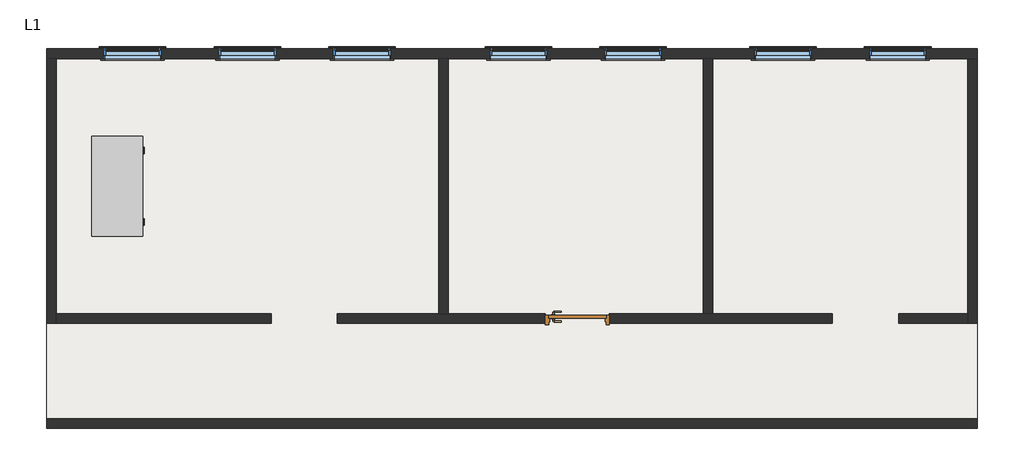
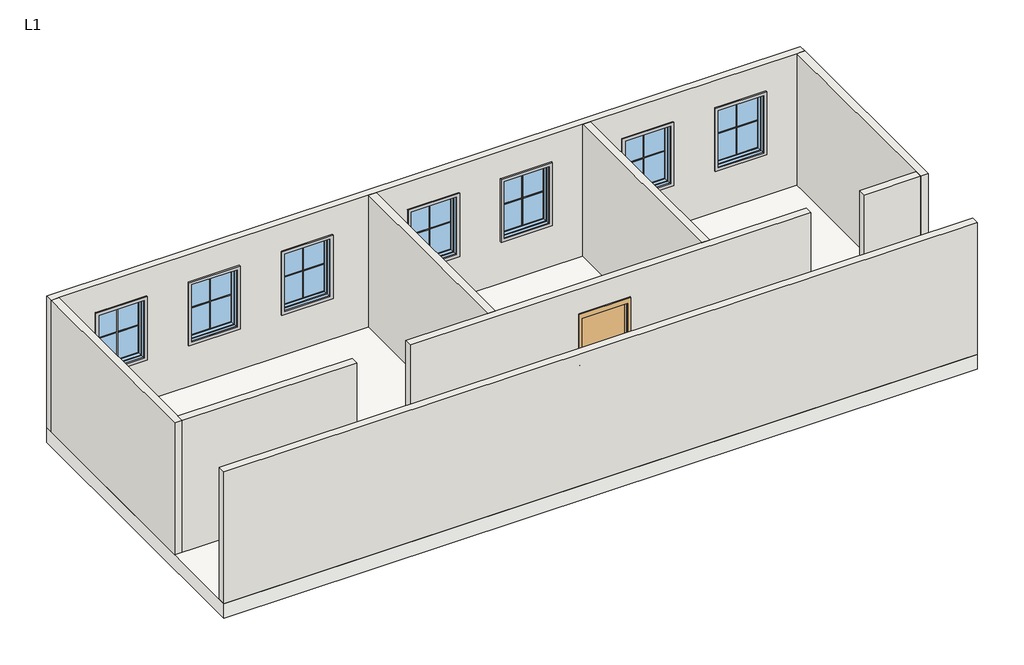
# One storey: 21 proxies, 9 walls, 7 windows, 1 door, 1 furniture element, 1 slab.
"""IFC4 building model written with IfcOpenShell, lengths in millimetres."""

import ifcopenshell
import ifcopenshell.guid

model = None  # the IFC model being written
_history = None  # IfcOwnerHistory: only IFC2X3 demands one
_inside = {}  # id of a spatial element -> (the spatial element, [elements in it])
_under = {}  # id of a project, library or spatial element -> (it, [spatial elements below it])
_declared = {}  # id of a project -> (the project, [libraries it declares])
_typed = {}  # id of a type object -> (the type object, [elements of that type])
_made_of = {}  # id of a material, layer set ... -> (it, [elements and type objects made of it])


def new_model(schema):
    """Start an empty IFC model of exactly this schema.

    Asked for "IFC4X3", IfcOpenShell would pick the latest addendum, in which some entities
    have other attributes; the version numbers below select the first issue.
    IFC2X3 requires an IfcOwnerHistory on every rooted entity: one is made here for all.
    """
    global model, _history
    if schema == "IFC4X3":
        model = ifcopenshell.file(schema_version=(4, 3, 0, 0))
    else:
        model = ifcopenshell.file(schema=schema)
    _inside.clear()
    _under.clear()
    _declared.clear()
    _typed.clear()
    _made_of.clear()
    _history = None
    if model.schema == "IFC2X3":
        org = make("IfcOrganization", Name="unknown")
        user = make(
            "IfcPersonAndOrganization",
            ThePerson=make("IfcPerson", FamilyName="unknown"),
            TheOrganization=org,
        )
        app = make(
            "IfcApplication",
            ApplicationDeveloper=org,
            Version="unknown",
            ApplicationFullName="unknown",
            ApplicationIdentifier="unknown",
        )
        _history = make(
            "IfcOwnerHistory",
            OwningUser=user,
            OwningApplication=app,
            ChangeAction="ADDED",
            CreationDate=0,
        )
    return model


def make(cls, **values):
    """One entity of the class cls with the attributes given. An attribute that is None is left unset."""
    return model.create_entity(
        cls, **{name: value for name, value in values.items() if value is not None}
    )


def rooted(cls, **values):
    """An entity with a GlobalId (a new one), such as an element, a storey or a relation."""
    return make(cls, GlobalId=ifcopenshell.guid.new(), OwnerHistory=_history, **values)


def si_unit(unit_type, name, prefix=None):
    """IfcSIUnit, for example si_unit("LENGTHUNIT", "METRE", prefix="MILLI")."""
    return make("IfcSIUnit", UnitType=unit_type, Prefix=prefix, Name=name)


def assignment(units):
    """IfcUnitAssignment: the units of a project."""
    return None if units is None else make("IfcUnitAssignment", Units=units)


def point(xyz):
    """IfcCartesianPoint."""
    return None if xyz is None else make("IfcCartesianPoint", Coordinates=xyz)


def direction(xyz):
    """IfcDirection."""
    return None if xyz is None else make("IfcDirection", DirectionRatios=xyz)


def frame(location, z_axis=None, x_axis=None):
    """IfcAxis2Placement3D, a coordinate frame: its origin and axes. An axis left out is left unset."""
    return make(
        "IfcAxis2Placement3D",
        Location=point(location),
        Axis=direction(z_axis),
        RefDirection=direction(x_axis),
    )


def frame_2d(location, x_axis=None):
    """IfcAxis2Placement2D, a coordinate frame in the plane: its origin and x axis."""
    return make(
        "IfcAxis2Placement2D", Location=point(location), RefDirection=direction(x_axis)
    )


def origin():
    """The frame at (0, 0, 0) with its axes left unset."""
    return frame((0.0, 0.0, 0.0))


def origin_with_axes():
    """The frame at (0, 0, 0) with the z axis (0, 0, 1) and the x axis (1, 0, 0) written out."""
    return frame((0.0, 0.0, 0.0), z_axis=(0.0, 0.0, 1.0), x_axis=(1.0, 0.0, 0.0))


def place(relative_to, where):
    """IfcLocalPlacement: puts the frame where relative to a parent placement (None: the world)."""
    return make(
        "IfcLocalPlacement", PlacementRelTo=relative_to, RelativePlacement=where
    )


def context(
    kind, dimensions, precision=None, world=None, true_north=None, identifier=None
):
    """IfcGeometricRepresentationContext, for example the 3D "Model" context."""
    return make(
        "IfcGeometricRepresentationContext",
        ContextIdentifier=identifier,
        ContextType=kind,
        CoordinateSpaceDimension=dimensions,
        Precision=precision,
        WorldCoordinateSystem=world,
        TrueNorth=true_north,
    )


def project(units=None, contexts=None):
    """IfcProject with its units and contexts."""
    return rooted(
        "IfcProject",
        Name="project",
        RepresentationContexts=contexts,
        UnitsInContext=assignment(units),
    )


def spatial(cls, under=None, at=None, **own):
    """A site, building, storey or space (cls), placed at a placement, below another one or the project."""
    s = rooted(cls, ObjectPlacement=at, **own)
    if under is not None:
        _under.setdefault(under.id(), (under, []))[1].append(s)
    return s


def polyline(points):
    """IfcPolyline through the points."""
    return make("IfcPolyline", Points=[point(p) for p in points])


def circle_curve(where, radius):
    """IfcCircle in the frame where."""
    return make("IfcCircle", Position=where, Radius=radius)


def ellipse_curve(where, semi_axis1, semi_axis2):
    """IfcEllipse in the frame where."""
    return make(
        "IfcEllipse", Position=where, SemiAxis1=semi_axis1, SemiAxis2=semi_axis2
    )


def trimmed(basis, trim1, trim2, sense, master):
    """IfcTrimmedCurve: the piece of a basis curve between two trims."""
    return make(
        "IfcTrimmedCurve",
        BasisCurve=basis,
        Trim1=trim1,
        Trim2=trim2,
        SenseAgreement=sense,
        MasterRepresentation=master,
    )


def segment(curve, same_sense, transition):
    """IfcCompositeCurveSegment."""
    return make(
        "IfcCompositeCurveSegment",
        Transition=transition,
        SameSense=same_sense,
        ParentCurve=curve,
    )


def composite_curve(segments, self_intersect=None):
    """IfcCompositeCurve: segments joined end to end."""
    return make("IfcCompositeCurve", Segments=segments, SelfIntersect=self_intersect)


def outline(outer, holes=None, kind="AREA"):
    """IfcArbitraryClosedProfileDef: a profile drawn as a closed curve; with holes, ...WithVoids."""
    if holes is None:
        return make("IfcArbitraryClosedProfileDef", ProfileType=kind, OuterCurve=outer)
    return make(
        "IfcArbitraryProfileDefWithVoids",
        ProfileType=kind,
        OuterCurve=outer,
        InnerCurves=holes,
    )


def extrude(swept, where, along, depth):
    """IfcExtrudedAreaSolid: the profile swept, set in the frame where, extruded along a direction by depth."""
    return make(
        "IfcExtrudedAreaSolid",
        SweptArea=swept,
        Position=where,
        ExtrudedDirection=direction(along),
        Depth=depth,
    )


def faces_of(points, faces, orient=None, outer=None):
    """IfcFace entities. A face is a list of loops; a loop is a list of indices into points, from 0.

    orient and outer hold one flag for each loop. By default every Orientation is true, the
    first loop of a face is its IfcFaceOuterBound and the others are IfcFaceBound.
    """
    made = []
    for i, loops in enumerate(faces):
        bounds = []
        for j, loop in enumerate(loops):
            is_outer = j == 0 if outer is None else outer[i][j]
            bounds.append(
                make(
                    "IfcFaceOuterBound" if is_outer else "IfcFaceBound",
                    Bound=make("IfcPolyLoop", Polygon=[points[k] for k in loop]),
                    Orientation=True if orient is None else orient[i][j],
                )
            )
        made.append(make("IfcFace", Bounds=bounds))
    return made


def faceted_brep(points, faces, orient=None, outer=None, voids=None):
    """IfcFacetedBrep: a solid bounded by flat faces; with voids (closed shells), ...WithVoids."""
    shared = [point(p) for p in points]
    hull = make("IfcClosedShell", CfsFaces=faces_of(shared, faces, orient, outer))
    if voids is None:
        return make("IfcFacetedBrep", Outer=hull)
    return make(
        "IfcFacetedBrepWithVoids",
        Outer=hull,
        Voids=[
            make(cls, CfsFaces=faces_of(shared, fs, o, b)) for cls, fs, o, b in voids
        ],
    )


def shape(context_of_items, identifier, shape_type, items):
    """IfcShapeRepresentation: the items that make up one representation, for example the "Body"."""
    return make(
        "IfcShapeRepresentation",
        ContextOfItems=context_of_items,
        RepresentationIdentifier=identifier,
        RepresentationType=shape_type,
        Items=items,
    )


def source(mapping_origin, context_of_items, identifier, shape_type, items):
    """IfcRepresentationMap: a shape defined once, which mapped items show again and again."""
    return make(
        "IfcRepresentationMap",
        MappingOrigin=mapping_origin,
        MappedRepresentation=shape(context_of_items, identifier, shape_type, items),
    )


def transform(
    local_origin,
    x_axis=None,
    y_axis=None,
    z_axis=None,
    scale=None,
    scale2=None,
    scale3=None,
    uniform=True,
):
    """IfcCartesianTransformationOperator3D, or its non-uniform kind. x_axis, y_axis, z_axis: its Axis1, 2, 3."""
    if uniform:
        return make(
            "IfcCartesianTransformationOperator3D",
            Axis1=direction(x_axis),
            Axis2=direction(y_axis),
            LocalOrigin=point(local_origin),
            Scale=scale,
            Axis3=direction(z_axis),
        )
    return make(
        "IfcCartesianTransformationOperator3DnonUniform",
        Axis1=direction(x_axis),
        Axis2=direction(y_axis),
        LocalOrigin=point(local_origin),
        Scale=scale,
        Axis3=direction(z_axis),
        Scale2=scale2,
        Scale3=scale3,
    )


def mapped(mapping_source, mapping_target):
    """IfcMappedItem: shows the shape of a source again, moved by a transform."""
    return make(
        "IfcMappedItem", MappingSource=mapping_source, MappingTarget=mapping_target
    )


def made_of(thing, what):
    """Note that an element or type object is made of a material, layer set ...; save() writes the relation."""
    if what is not None:
        _made_of.setdefault(what.id(), (what, []))[1].append(thing)
    return thing


def element(
    cls,
    number,
    at=None,
    inside=None,
    cuts=None,
    type_object=None,
    material=None,
    context=None,
    identifier="Body",
    shape_type=None,
    held_by="IfcProductDefinitionShape",
    body=None,
    shapes=None,
    **own,
):
    """One element of the class cls, such as IfcWall. Its Tag is "e" and its number.

    at: its placement. inside: the storey or other place that contains it. cuts: it is an
    opening in that element (IfcRelVoidsElement). A single representation is given by context,
    identifier, shape_type and body (its items); several are given by shapes. held_by: the class
    of the entity that holds the representations. save() writes the other relations.
    """
    e = rooted(cls, Tag="e%d" % number, ObjectPlacement=at, **own)
    if body is not None:
        shapes = [shape(context, identifier, shape_type, body)]
    if shapes is not None:
        e.Representation = make(held_by, Representations=shapes)
    if inside is not None:
        _inside.setdefault(inside.id(), (inside, []))[1].append(e)
    if cuts is not None:
        rooted(
            "IfcRelVoidsElement", RelatingBuildingElement=cuts, RelatedOpeningElement=e
        )
    if type_object is not None:
        _typed.setdefault(type_object.id(), (type_object, []))[1].append(e)
    return made_of(e, material)


def aggregate(whole, parts):
    """IfcRelAggregates: a whole, such as a stair, and the parts it consists of."""
    return rooted("IfcRelAggregates", RelatingObject=whole, RelatedObjects=parts)


def save(model, path):
    """Write the relations noted so far, then the file.

    IfcRelAggregates (storeys below a building ...), IfcRelContainedInSpatialStructure (elements
    in a storey), IfcRelDefinesByType, IfcRelAssociatesMaterial and IfcRelDeclares: one each for
    every whole, place, type object, material and project.
    """
    for whole, parts in _under.values():
        aggregate(whole, parts)
    for where, things in _inside.values():
        rooted(
            "IfcRelContainedInSpatialStructure",
            RelatedElements=things,
            RelatingStructure=where,
        )
    for kind, things in _typed.values():
        rooted("IfcRelDefinesByType", RelatedObjects=things, RelatingType=kind)
    for what, things in _made_of.values():
        rooted("IfcRelAssociatesMaterial", RelatedObjects=things, RelatingMaterial=what)
    for by, libraries in _declared.values():
        rooted("IfcRelDeclares", RelatingContext=by, RelatedDefinitions=libraries)
    model.write(path)


def plane_surface(at):
    """IfcPlane: the flat surface through the origin of the frame at, square to its z axis."""
    return make("IfcPlane", Position=at)


def cylinder_surface(at, radius):
    """IfcCylindricalSurface: all points at the distance radius from the z axis of the frame at."""
    return make("IfcCylindricalSurface", Position=at, Radius=radius)


def revolved_surface(curve, axis_point, axis_direction):
    """IfcSurfaceOfRevolution: the curve turned about the line through axis_point along axis_direction."""
    return make(
        "IfcSurfaceOfRevolution",
        SweptCurve=make("IfcArbitraryOpenProfileDef", ProfileType="CURVE", Curve=curve),
        AxisPosition=make("IfcAxis1Placement", Location=point(axis_point), Axis=direction(axis_direction)),
    )


def advanced_brep(points, edges, surfaces, faces):
    """IfcAdvancedBrep: a solid bounded by faces that lie on surfaces and meet in shared edges.

    An edge is (start, end): straight between two places in points (the first is 0);
    or (start, end, curve); or (start, end, curve, False) where it runs against its curve.
    A face is (place in surfaces, loops), or (place, loops, False) where it looks against
    its surface's normal. A loop lists edges by number (the first is 1), with a minus sign
    where the edge is run from its end to its start. The first loop is the outer one.
    """
    corners = [point(p) for p in points]
    vertices = [make("IfcVertexPoint", VertexGeometry=c) for c in corners]
    made = []
    for start, end, *more in edges:
        made.append(
            make(
                "IfcEdgeCurve",
                EdgeStart=vertices[start],
                EdgeEnd=vertices[end],
                EdgeGeometry=more[0] if more else make("IfcPolyline", Points=[corners[start], corners[end]]),
                SameSense=more[1] if len(more) > 1 else True,
            )
        )
    hull = []
    for where, loops, *sense in faces:
        bounds = []
        for j, loop in enumerate(loops):
            ring = [make("IfcOrientedEdge", EdgeElement=made[abs(k) - 1], Orientation=k > 0) for k in loop]
            bounds.append(
                make(
                    "IfcFaceOuterBound" if j == 0 else "IfcFaceBound",
                    Bound=make("IfcEdgeLoop", EdgeList=ring),
                    Orientation=True,
                )
            )
        hull.append(make("IfcAdvancedFace", Bounds=bounds, FaceSurface=surfaces[where], SameSense=sense[0] if sense else True))
    return make("IfcAdvancedBrep", Outer=make("IfcClosedShell", CfsFaces=hull))


def m_muntin_pattern_2x2_m_muntin_pattern_2x2_ad852c99(model_context):
    return source(origin(), model_context, "Body", "SweptSolid", [
        extrude(outline(polyline([(568.25, -6.35), (568.25, -411.9), (555.55, -411.9), (555.55, -6.35), (0.0, -6.35), (0.0, 6.35), (555.55, 6.35), (555.55, 411.9), (568.25, 411.9), (568.25, 6.35), (1123.8, 6.35), (1123.8, -6.35), (568.25, -6.35)])), frame((0.0, -22.225, 0.0), z_axis=(0.0, 1.0, 0.0), x_axis=(0.0, 0.0, 1.0)), (0.0, 0.0, 1.0), 12.7),
        extrude(outline(polyline([(568.25, -6.35), (568.25, -411.9), (555.55, -411.9), (555.55, -6.35), (0.0, -6.35), (0.0, 6.35), (555.55, 6.35), (555.55, 411.9), (568.25, 411.9), (568.25, 6.35), (1123.8, 6.35), (1123.8, -6.35), (568.25, -6.35)])), frame((0.0, 9.525, 0.0), z_axis=(0.0, 1.0, 0.0), x_axis=(0.0, 0.0, 1.0)), (0.0, 0.0, 1.0), 12.7),
    ])


def m_trim_window_exterior_flat_with_sill_71544b40(model_context):
    return source(origin(), model_context, "Body", "SweptSolid", [
        extrude(outline(polyline([(510.0, -1220.4323709), (510.0, -1280.4323709), (-510.0, -1280.4323709), (-510.0, -1220.4323709), (510.0, -1220.4323709)])), origin_with_axes(), (0.0, 0.0, 1.0), 19.05),
        extrude(outline(polyline([(-1230.0, 38.1), (-1202.4580645, 38.1), (-1200.0, 19.05), (-1200.0, 0.0), (-1220.4323709, 0.0), (-1220.4323709, 19.05), (-1230.0, 19.05), (-1230.0, 38.1)])), frame((-522.7, 0.0, 0.0), z_axis=(1.0, 0.0, 0.0), x_axis=(0.0, 1.0, 0.0)), (0.0, 0.0, 1.0), 1045.4),
        extrude(outline(polyline([(-510.0, 60.0), (510.0, 60.0), (510.0, -1200.0), (450.0, -1200.0), (450.0, 0.0), (-450.0, 0.0), (-450.0, -1200.0), (-510.0, -1200.0), (-510.0, 60.0)])), origin_with_axes(), (0.0, 0.0, 1.0), 19.05),
    ])


def m_trim_window_interior_flat_picture_frame_24fe8ef8(model_context):
    return source(origin(), model_context, "Body", "SweptSolid", [
        extrude(outline(polyline([(497.3, 47.3), (497.3, -1247.3), (-497.3, -1247.3), (-497.3, 47.3), (497.3, 47.3)]), holes=[polyline([(437.3, -12.7), (-437.3, -12.7), (-437.3, -1187.3), (437.3, -1187.3), (437.3, -12.7)])]), origin_with_axes(), (0.0, 0.0, 1.0), 30.0),
    ])


def m_door_passage_single_flush_900_x_2100mm_f70d95c9(model_context):
    return source(origin(), model_context, "Body", "SolidModel", [
        advanced_brep(
        [(-384.990625, 3.35, 1000.0), (-364.990625, 3.35, 1000.0), (-364.990625, -26.65, 1000.0), (-384.990625, -26.65, 1000.0), (-359.990625, -31.65, 1000.0), (-359.990625, -51.65, 1000.0), (-254.990625, -51.65, 1000.0), (-254.990625, -31.65, 1000.0)],
        [
            (0, 1, circle_curve(frame((-374.990625, 3.35, 1000.0), z_axis=(0.0, 1.0, 0.0), x_axis=(1.0, 0.0, 0.0)), 10.0)),
            (1, 0, circle_curve(frame((-374.990625, 3.35, 1000.0), z_axis=(0.0, 1.0, 0.0), x_axis=(1.0, 0.0, 0.0)), 10.0)),
            (1, 2),
            (2, 3, circle_curve(frame((-374.990625, -26.65, 1000.0), z_axis=(0.0, 1.0, 0.0), x_axis=(1.0, 0.0, 0.0)), 10.0)),
            (3, 0),
            (3, 2, circle_curve(frame((-374.990625, -26.65, 1000.0), z_axis=(0.0, 1.0, 0.0), x_axis=(1.0, 0.0, 0.0)), 10.0)),
            (4, 5, circle_curve(frame((-359.990625, -41.65, 1000.0), z_axis=(-1.0, 0.0, 0.0), x_axis=(0.0, 1.0, 0.0)), 10.0)),
            (5, 3, circle_curve(frame((-359.990625, -26.65, 1000.0), z_axis=(0.0, 0.0, -1.0), x_axis=(-1.0, 0.0, 0.0)), 25.0)),
            (2, 4, circle_curve(frame((-359.990625, -26.65, 1000.0), z_axis=(0.0, 0.0, 1.0), x_axis=(-1.0, 0.0, 0.0)), 5.0)),
            (5, 4, circle_curve(frame((-359.990625, -41.65, 1000.0), z_axis=(-1.0, 0.0, 0.0), x_axis=(0.0, 1.0, 0.0)), 10.0)),
            (6, 7, circle_curve(frame((-254.990625, -41.65, 1000.0), z_axis=(1.0, 0.0, 0.0), x_axis=(0.0, 1.0, 0.0)), 10.0)),
            (7, 6, circle_curve(frame((-254.990625, -41.65, 1000.0), z_axis=(1.0, 0.0, 0.0), x_axis=(0.0, 1.0, 0.0)), 10.0)),
            (4, 7),
            (6, 5),
        ],
        [
            plane_surface(frame((-374.990625, 3.35, 1000.0), z_axis=(0.0, 1.0, 0.0), x_axis=(0.0, 0.0, 1.0))),
            cylinder_surface(frame((-374.990625, 3.35, 1000.0), z_axis=(0.0, 1.0, 0.0), x_axis=(1.0, 0.0, 0.0)), 10.0),
            revolved_surface(trimmed(ellipse_curve(frame((-374.990625, -26.65, 1000.0), z_axis=(0.0, -1.0, 0.0), x_axis=(1.0, 0.0, 0.0)), 10.0, 10.0), [point((-384.990625, -26.65, 1000.0))], [point((-364.990625, -26.65, 1000.0))], True, "CARTESIAN"), (-359.990625, -26.65, 1000.0), (0.0, 0.0, -1.0)),
            revolved_surface(trimmed(ellipse_curve(frame((-374.990625, -26.65, 1000.0), z_axis=(0.0, -1.0, 0.0), x_axis=(1.0, 0.0, 0.0)), 10.0, 10.0), [point((-364.990625, -26.65, 1000.0))], [point((-384.990625, -26.65, 1000.0))], True, "CARTESIAN"), (-359.990625, -26.65, 1000.0), (0.0, 0.0, -1.0)),
            plane_surface(frame((-254.990625, -41.65, 1000.0), z_axis=(1.0, 0.0, 0.0), x_axis=(0.0, 0.0, 1.0))),
            cylinder_surface(frame((-359.990625, -41.65, 1000.0), z_axis=(-1.0, 0.0, 0.0), x_axis=(0.0, 1.0, 0.0)), 10.0),
        ],
        [
            (0, [[1, 2]]),
            (1, [[3, 4, 5, -2]]),
            (1, [[-5, 6, -3, -1]]),
            (2, [[7, 8, -4, 9]]),
            (3, [[10, -9, -6, -8]]),
            (4, [[11, 12]]),
            (5, [[13, -11, 14, -7]]),
            (5, [[-14, -12, -13, -10]]),
        ],
    ),
        extrude(outline(composite_curve([segment(trimmed(circle_curve(frame_2d((1000.0, -377.490625)), 30.0), [point((1000.0, -407.490625))], [point((1000.0, -347.490625))], False, "CARTESIAN"), True, "CONTINUOUS"), segment(trimmed(circle_curve(frame_2d((1000.0, -377.490625)), 30.0), [point((1000.0, -347.490625))], [point((1000.0, -407.490625))], False, "CARTESIAN"), True, "CONTINUOUS")], self_intersect=False)), frame((0.0, 3.35, 0.0), z_axis=(0.0, 1.0, 0.0), x_axis=(0.0, 0.0, 1.0)), (0.0, 0.0, 1.0), 8.0),
        advanced_brep(
        [(-384.990625, 64.35, 1000.0), (-364.990625, 64.35, 1000.0), (-384.990625, 94.35, 1000.0), (-364.990625, 94.35, 1000.0), (-359.990625, 99.35, 1000.0), (-359.990625, 119.35, 1000.0), (-254.990625, 119.35, 1000.0), (-254.990625, 99.35, 1000.0)],
        [
            (0, 1, circle_curve(frame((-374.990625, 64.35, 1000.0), z_axis=(0.0, -1.0, 0.0), x_axis=(1.0, 0.0, 0.0)), 10.0)),
            (1, 0, circle_curve(frame((-374.990625, 64.35, 1000.0), z_axis=(0.0, -1.0, 0.0), x_axis=(1.0, 0.0, 0.0)), 10.0)),
            (0, 2),
            (2, 3, circle_curve(frame((-374.990625, 94.35, 1000.0), z_axis=(0.0, -1.0, 0.0), x_axis=(1.0, 0.0, 0.0)), 10.0)),
            (3, 1),
            (3, 2, circle_curve(frame((-374.990625, 94.35, 1000.0), z_axis=(0.0, -1.0, 0.0), x_axis=(1.0, 0.0, 0.0)), 10.0)),
            (4, 3, circle_curve(frame((-359.990625, 94.35, 1000.0), z_axis=(0.0, 0.0, 1.0), x_axis=(-1.0, 0.0, 0.0)), 5.0)),
            (2, 5, circle_curve(frame((-359.990625, 94.35, 1000.0), z_axis=(0.0, 0.0, -1.0), x_axis=(-1.0, 0.0, 0.0)), 25.0)),
            (5, 4, circle_curve(frame((-359.990625, 109.35, 1000.0), z_axis=(-1.0, 0.0, 0.0), x_axis=(0.0, -1.0, 0.0)), 10.0)),
            (4, 5, circle_curve(frame((-359.990625, 109.35, 1000.0), z_axis=(-1.0, 0.0, 0.0), x_axis=(0.0, -1.0, 0.0)), 10.0)),
            (6, 7, circle_curve(frame((-254.990625, 109.35, 1000.0), z_axis=(1.0, 0.0, 0.0), x_axis=(0.0, -1.0, 0.0)), 10.0)),
            (7, 6, circle_curve(frame((-254.990625, 109.35, 1000.0), z_axis=(1.0, 0.0, 0.0), x_axis=(0.0, -1.0, 0.0)), 10.0)),
            (5, 6),
            (7, 4),
        ],
        [
            plane_surface(frame((-374.990625, 64.35, 1000.0), z_axis=(0.0, -1.0, 0.0), x_axis=(0.0, 0.0, 1.0))),
            cylinder_surface(frame((-374.990625, 64.35, 1000.0), z_axis=(0.0, -1.0, 0.0), x_axis=(1.0, 0.0, 0.0)), 10.0),
            revolved_surface(trimmed(ellipse_curve(frame((-374.990625, 94.35, 1000.0), z_axis=(0.0, -1.0, 0.0), x_axis=(1.0, 0.0, 0.0)), 10.0, 10.0), [point((-384.990625, 94.35, 1000.0))], [point((-364.990625, 94.35, 1000.0))], True, "CARTESIAN"), (-359.990625, 94.35, 1000.0), (0.0, 0.0, -1.0)),
            revolved_surface(trimmed(ellipse_curve(frame((-374.990625, 94.35, 1000.0), z_axis=(0.0, -1.0, 0.0), x_axis=(1.0, 0.0, 0.0)), 10.0, 10.0), [point((-364.990625, 94.35, 1000.0))], [point((-384.990625, 94.35, 1000.0))], True, "CARTESIAN"), (-359.990625, 94.35, 1000.0), (0.0, 0.0, -1.0)),
            plane_surface(frame((-254.990625, 109.35, 1000.0), z_axis=(1.0, 0.0, 0.0), x_axis=(0.0, 0.0, 1.0))),
            cylinder_surface(frame((-359.990625, 109.35, 1000.0), z_axis=(-1.0, 0.0, 0.0), x_axis=(0.0, -1.0, 0.0)), 10.0),
        ],
        [
            (0, [[1, 2]]),
            (1, [[-1, 3, 4, 5]]),
            (1, [[-2, -5, 6, -3]]),
            (2, [[7, -4, 8, 9]]),
            (3, [[-8, -6, -7, 10]]),
            (4, [[11, 12]]),
            (5, [[-9, 13, -12, 14]]),
            (5, [[-10, -14, -11, -13]]),
        ],
    ),
        extrude(outline(composite_curve([segment(trimmed(circle_curve(frame_2d((1000.0, -377.490625)), 30.0), [point((1000.0, -407.490625))], [point((1000.0, -347.490625))], False, "CARTESIAN"), True, "CONTINUOUS"), segment(trimmed(circle_curve(frame_2d((1000.0, -377.490625)), 30.0), [point((1000.0, -347.490625))], [point((1000.0, -407.490625))], False, "CARTESIAN"), True, "CONTINUOUS")], self_intersect=False)), frame((0.0, 56.35, 0.0), z_axis=(0.0, 1.0, 0.0), x_axis=(0.0, 0.0, 1.0)), (0.0, 0.0, 1.0), 8.0),
        extrude(outline(polyline([(450.0, 11.35), (-450.0, 11.35), (-450.0, 56.35), (450.0, 56.35), (450.0, 11.35)])), origin_with_axes(), (0.0, 0.0, 1.0), 2100.0),
        faceted_brep([(450.0, 6.5875, 0.0), (450.0, 56.35, 0.0), (500.0, 56.35, 0.0), (500.0, -93.65, 0.0), (450.0, -93.65, 0.0), (450.0, -44.4375, 0.0), (434.125, -44.4375, 0.0), (434.125, 6.5875, 0.0), (450.0, 6.5875, 2100.0), (450.0, 56.35, 2100.0), (-450.0, 56.35, 2100.0), (-450.0, 56.35, 0.0), (-500.0, 56.35, 0.0), (-500.0, 56.35, 2200.0), (500.0, 56.35, 2200.0), (500.0, -93.65, 2200.0), (-500.0, -93.65, 2200.0), (-500.0, -93.65, 0.0), (-450.0, -93.65, 0.0), (-450.0, -93.65, 2100.0), (450.0, -93.65, 2100.0), (450.0, -44.4375, 2100.0), (-450.0, -44.4375, 2100.0), (-450.0, -44.4375, 0.0), (-434.125, -44.4375, 0.0), (-434.125, -44.4375, 2084.125), (434.125, -44.4375, 2084.125), (434.125, 6.5875, 2084.125), (-434.125, 6.5875, 2084.125), (-434.125, 6.5875, 0.0), (-450.0, 6.5875, 0.0), (-450.0, 6.5875, 2100.0)], [[[0, 1, 2, 3, 4, 5, 6, 7]], [[1, 0, 8, 9]], [[2, 1, 9, 10, 11, 12, 13, 14]], [[3, 2, 14, 15]], [[4, 3, 15, 16, 17, 18, 19, 20]], [[5, 4, 20, 21]], [[6, 5, 21, 22, 23, 24, 25, 26]], [[7, 6, 26, 27]], [[0, 7, 27, 28, 29, 30, 31, 8]], [[9, 8, 31, 10]], [[20, 19, 22, 21]], [[26, 25, 28, 27]], [[12, 11, 30, 29, 24, 23, 18, 17]], [[11, 10, 31, 30]], [[13, 12, 17, 16]], [[19, 18, 23, 22]], [[25, 24, 29, 28]], [[15, 14, 13, 16]]]),
    ])


def m_desk_1525_x_762mm_student_34485ced(model_context):
    return source(origin(), model_context, "Body", "SolidModel", [
        extrude(outline(polyline([(1118.1, 0.0), (1118.1, 635.0), (405.9, 635.0), (405.9, 0.0), (-0.5, 0.0), (-0.5, 762.0), (1524.5, 762.0), (1524.5, 0.0), (1118.1, 0.0)])), frame((0.0, 0.0, 152.0), z_axis=(0.0, 0.0, 1.0), x_axis=(1.0, 0.0, 0.0)), (0.0, 0.0, 1.0), 571.9),
        extrude(outline(polyline([(-19.55, -19.05), (-19.55, 781.05), (1543.55, 781.05), (1543.55, -19.05), (-19.55, -19.05)])), frame((0.0, 0.0, 723.9), z_axis=(0.0, 0.0, 1.0), x_axis=(1.0, 0.0, 0.0)), (0.0, 0.0, 1.0), 38.1),
        faceted_brep([(1422.9, 0.0, 152.0), (1524.5, 0.0, 152.0), (1524.5, 101.6, 152.0), (1422.9, 101.6, 152.0), (1448.3, 0.0, 0.0), (1448.3, 76.2, 0.0), (1524.5, 76.2, 0.0), (1524.5, 0.0, 0.0)], [[[0, 1, 2, 3]], [[4, 5, 6, 7]], [[4, 7, 1, 0]], [[7, 6, 2, 1]], [[6, 5, 3, 2]], [[5, 4, 0, 3]]]),
        faceted_brep([(1422.9, 762.0, 152.0), (1422.9, 660.4, 152.0), (1524.5, 660.4, 152.0), (1524.5, 762.0, 152.0), (1448.3, 762.0, 0.0), (1524.5, 762.0, 0.0), (1524.5, 685.8, 0.0), (1448.3, 685.8, 0.0)], [[[0, 1, 2, 3]], [[4, 5, 6, 7]], [[4, 7, 1, 0]], [[7, 6, 2, 1]], [[6, 5, 3, 2]], [[5, 4, 0, 3]]]),
        faceted_brep([(101.1, 762.0, 152.0), (-0.5, 762.0, 152.0), (-0.5, 660.4, 152.0), (101.1, 660.4, 152.0), (75.7, 762.0, 0.0), (75.7, 685.8, 0.0), (-0.5, 685.8, 0.0), (-0.5, 762.0, 0.0)], [[[0, 1, 2, 3]], [[4, 5, 6, 7]], [[4, 7, 1, 0]], [[7, 6, 2, 1]], [[6, 5, 3, 2]], [[5, 4, 0, 3]]]),
        faceted_brep([(101.1, 0.0, 152.0), (101.1, 101.6, 152.0), (-0.5, 101.6, 152.0), (-0.5, 0.0, 152.0), (75.7, 0.0, 0.0), (-0.5, 0.0, 0.0), (-0.5, 76.2, 0.0), (75.7, 76.2, 0.0)], [[[0, 1, 2, 3]], [[4, 5, 6, 7]], [[4, 7, 1, 0]], [[7, 6, 2, 1]], [[6, 5, 3, 2]], [[5, 4, 0, 3]]]),
        extrude(outline(polyline([(1137.15, 0.0), (1505.45, 0.0), (1505.45, -12.7), (1137.15, -12.7), (1137.15, 0.0)])), frame((0.0, 0.0, 602.85), z_axis=(0.0, 0.0, 1.0), x_axis=(1.0, 0.0, 0.0)), (0.0, 0.0, 1.0), 102.0),
        extrude(outline(polyline([(1137.15, 0.0), (1505.45, 0.0), (1505.45, -12.7), (1137.15, -12.7), (1137.15, 0.0)])), frame((0.0, 0.0, 171.05), z_axis=(0.0, 0.0, 1.0), x_axis=(1.0, 0.0, 0.0)), (0.0, 0.0, 1.0), 171.45),
        extrude(outline(polyline([(1137.15, 0.0), (1505.45, 0.0), (1505.45, -12.7), (1137.15, -12.7), (1137.15, 0.0)])), frame((0.0, 0.0, 482.2), z_axis=(0.0, 0.0, 1.0), x_axis=(1.0, 0.0, 0.0)), (0.0, 0.0, 1.0), 101.6),
        extrude(outline(polyline([(1137.15, 0.0), (1505.45, 0.0), (1505.45, -12.7), (1137.15, -12.7), (1137.15, 0.0)])), frame((0.0, 0.0, 361.55), z_axis=(0.0, 0.0, 1.0), x_axis=(1.0, 0.0, 0.0)), (0.0, 0.0, 1.0), 101.6),
        extrude(outline(polyline([(18.55, 0.0), (386.85, 0.0), (386.85, -12.7), (18.55, -12.7), (18.55, 0.0)])), frame((0.0, 0.0, 603.25), z_axis=(0.0, 0.0, 1.0), x_axis=(1.0, 0.0, 0.0)), (0.0, 0.0, 1.0), 101.6),
        extrude(outline(polyline([(18.55, 0.0), (386.85, 0.0), (386.85, -12.7), (18.55, -12.7), (18.55, 0.0)])), frame((0.0, 0.0, 171.05), z_axis=(0.0, 0.0, 1.0), x_axis=(1.0, 0.0, 0.0)), (0.0, 0.0, 1.0), 413.15),
        faceted_brep([(1365.75, -12.7, 304.8), (1372.1, -12.7, 304.8), (1372.1, -12.7, 292.1), (1365.75, -12.7, 292.1), (1365.75, -31.75, 304.8), (1372.1, -38.1, 304.8), (1372.1, -38.1, 292.1), (1365.75, -31.75, 292.1), (1276.85, -31.75, 304.8), (1270.5, -38.1, 304.8), (1270.5, -38.1, 292.1), (1276.85, -31.75, 292.1), (1276.85, -12.7, 304.8), (1276.85, -12.7, 292.1), (1270.5, -12.7, 292.1), (1270.5, -12.7, 304.8)], [[[0, 1, 2, 3]], [[1, 0, 4, 5]], [[2, 1, 5, 6]], [[3, 2, 6, 7]], [[0, 3, 7, 4]], [[5, 4, 8, 9]], [[6, 5, 9, 10]], [[7, 6, 10, 11]], [[4, 7, 11, 8]], [[12, 13, 14, 15]], [[9, 8, 12, 15]], [[10, 9, 15, 14]], [[11, 10, 14, 13]], [[8, 11, 13, 12]]]),
        faceted_brep([(1365.75, -12.7, 425.45), (1372.1, -12.7, 425.45), (1372.1, -12.7, 412.75), (1365.75, -12.7, 412.75), (1365.75, -31.75, 425.45), (1372.1, -38.1, 425.45), (1372.1, -38.1, 412.75), (1365.75, -31.75, 412.75), (1276.85, -31.75, 425.45), (1270.5, -38.1, 425.45), (1270.5, -38.1, 412.75), (1276.85, -31.75, 412.75), (1276.85, -12.7, 425.45), (1276.85, -12.7, 412.75), (1270.5, -12.7, 412.75), (1270.5, -12.7, 425.45)], [[[0, 1, 2, 3]], [[1, 0, 4, 5]], [[2, 1, 5, 6]], [[3, 2, 6, 7]], [[0, 3, 7, 4]], [[5, 4, 8, 9]], [[6, 5, 9, 10]], [[7, 6, 10, 11]], [[4, 7, 11, 8]], [[12, 13, 14, 15]], [[9, 8, 12, 15]], [[10, 9, 15, 14]], [[11, 10, 14, 13]], [[8, 11, 13, 12]]]),
        faceted_brep([(1365.75, -12.7, 546.1), (1372.1, -12.7, 546.1), (1372.1, -12.7, 533.4), (1365.75, -12.7, 533.4), (1365.75, -31.75, 546.1), (1372.1, -38.1, 546.1), (1372.1, -38.1, 533.4), (1365.75, -31.75, 533.4), (1276.85, -31.75, 546.1), (1270.5, -38.1, 546.1), (1270.5, -38.1, 533.4), (1276.85, -31.75, 533.4), (1276.85, -12.7, 546.1), (1276.85, -12.7, 533.4), (1270.5, -12.7, 533.4), (1270.5, -12.7, 546.1)], [[[0, 1, 2, 3]], [[1, 0, 4, 5]], [[2, 1, 5, 6]], [[3, 2, 6, 7]], [[0, 3, 7, 4]], [[5, 4, 8, 9]], [[6, 5, 9, 10]], [[7, 6, 10, 11]], [[4, 7, 11, 8]], [[12, 13, 14, 15]], [[9, 8, 12, 15]], [[10, 9, 15, 14]], [[11, 10, 14, 13]], [[8, 11, 13, 12]]]),
        faceted_brep([(1365.75, -12.7, 666.75), (1372.1, -12.7, 666.75), (1372.1, -12.7, 654.05), (1365.75, -12.7, 654.05), (1365.75, -31.75, 666.75), (1372.1, -38.1, 666.75), (1372.1, -38.1, 654.05), (1365.75, -31.75, 654.05), (1276.85, -31.75, 666.75), (1270.5, -38.1, 666.75), (1270.5, -38.1, 654.05), (1276.85, -31.75, 654.05), (1276.85, -12.7, 666.75), (1276.85, -12.7, 654.05), (1270.5, -12.7, 654.05), (1270.5, -12.7, 666.75)], [[[0, 1, 2, 3]], [[1, 0, 4, 5]], [[2, 1, 5, 6]], [[3, 2, 6, 7]], [[0, 3, 7, 4]], [[5, 4, 8, 9]], [[6, 5, 9, 10]], [[7, 6, 10, 11]], [[4, 7, 11, 8]], [[12, 13, 14, 15]], [[9, 8, 12, 15]], [[10, 9, 15, 14]], [[11, 10, 14, 13]], [[8, 11, 13, 12]]]),
        faceted_brep([(158.25, -12.7, 546.1), (158.25, -12.7, 533.4), (151.9, -12.7, 533.4), (151.9, -12.7, 546.1), (158.25, -31.75, 546.1), (158.25, -31.75, 533.4), (151.9, -38.1, 533.4), (151.9, -38.1, 546.1), (247.15, -31.75, 546.1), (247.15, -31.75, 533.4), (253.5, -38.1, 533.4), (253.5, -38.1, 546.1), (247.15, -12.7, 546.1), (253.5, -12.7, 546.1), (253.5, -12.7, 533.4), (247.15, -12.7, 533.4)], [[[0, 1, 2, 3]], [[1, 0, 4, 5]], [[2, 1, 5, 6]], [[3, 2, 6, 7]], [[0, 3, 7, 4]], [[5, 4, 8, 9]], [[6, 5, 9, 10]], [[7, 6, 10, 11]], [[4, 7, 11, 8]], [[12, 13, 14, 15]], [[9, 8, 12, 15]], [[10, 9, 15, 14]], [[11, 10, 14, 13]], [[8, 11, 13, 12]]]),
        faceted_brep([(158.25, -12.7, 666.75), (158.25, -12.7, 654.05), (151.9, -12.7, 654.05), (151.9, -12.7, 666.75), (158.25, -31.75, 666.75), (158.25, -31.75, 654.05), (151.9, -38.1, 654.05), (151.9, -38.1, 666.75), (247.15, -31.75, 666.75), (247.15, -31.75, 654.05), (253.5, -38.1, 654.05), (253.5, -38.1, 666.75), (247.15, -12.7, 666.75), (253.5, -12.7, 666.75), (253.5, -12.7, 654.05), (247.15, -12.7, 654.05)], [[[0, 1, 2, 3]], [[1, 0, 4, 5]], [[2, 1, 5, 6]], [[3, 2, 6, 7]], [[0, 3, 7, 4]], [[5, 4, 8, 9]], [[6, 5, 9, 10]], [[7, 6, 10, 11]], [[4, 7, 11, 8]], [[12, 13, 14, 15]], [[9, 8, 12, 15]], [[10, 9, 15, 14]], [[11, 10, 14, 13]], [[8, 11, 13, 12]]]),
    ])


def m_window_fixed_900_x_1200mm_f2c8dc95(model_context):
    return source(origin(), model_context, "Body", "SolidModel", [
        faceted_brep([(450.0, -20.25, 2100.0), (450.0, 94.05, 2100.0), (-450.0, 94.05, 2100.0), (-450.0, -20.25, 2100.0), (-450.0, 94.05, 900.0), (-450.0, -20.25, 900.0), (450.0, 94.05, 900.0), (450.0, -20.25, 900.0), (418.25, -20.25, 2068.25), (418.25, -20.25, 931.75), (-418.25, -20.25, 931.75), (-418.25, -20.25, 2068.25), (-437.3, 94.05, 2087.3), (-437.3, 94.05, 912.7), (437.3, 94.05, 912.7), (437.3, 94.05, 2087.3), (418.25, 43.25, 2068.25), (-418.25, 43.25, 2068.25), (437.3, 43.25, 2087.3), (-437.3, 43.25, 2087.3), (-418.25, 43.25, 931.75), (-437.3, 43.25, 912.7), (418.25, 43.25, 931.75), (437.3, 43.25, 912.7)], [[[0, 1, 2, 3]], [[3, 2, 4, 5]], [[5, 4, 6, 7]], [[3, 5, 7, 0], [8, 9, 10, 11]], [[7, 6, 1, 0]], [[1, 6, 4, 2], [12, 13, 14, 15]], [[16, 8, 11, 17]], [[15, 18, 19, 12]], [[17, 11, 10, 20]], [[12, 19, 21, 13]], [[20, 10, 9, 22]], [[13, 21, 23, 14]], [[22, 9, 8, 16]], [[18, 23, 21, 19], [17, 20, 22, 16]], [[14, 23, 18, 15]]]),
        extrude(outline(polyline([(2100.0, -450.0), (900.0, -450.0), (900.0, 450.0), (2100.0, 450.0), (2100.0, -450.0)]), holes=[polyline([(2087.3, 437.3), (912.7, 437.3), (912.7, -437.3), (2087.3, -437.3), (2087.3, 437.3)])]), frame((0.0, -75.0, 0.0), z_axis=(0.0, 1.0, 0.0), x_axis=(0.0, 0.0, 1.0)), (0.0, 0.0, 1.0), 54.75),
        extrude(outline(polyline([(912.7, 437.3), (2087.3, 437.3), (2087.3, -437.3), (912.7, -437.3), (912.7, 437.3)]), holes=[polyline([(938.1, -411.9), (2061.9, -411.9), (2061.9, 411.9), (938.1, 411.9), (938.1, -411.9)])]), frame((0.0, 43.25, 0.0), z_axis=(0.0, 1.0, 0.0), x_axis=(0.0, 0.0, 1.0)), (0.0, 0.0, 1.0), 44.45),
        extrude(outline(polyline([(411.9, 75.0), (411.9, 68.65), (-411.9, 68.65), (-411.9, 75.0), (411.9, 75.0)])), frame((0.0, 0.0, 938.1), z_axis=(0.0, 0.0, 1.0), x_axis=(1.0, 0.0, 0.0)), (0.0, 0.0, 1.0), 1123.8),
        extrude(outline(polyline([(-411.9, 55.95), (-411.9, 62.3), (411.9, 62.3), (411.9, 55.95), (-411.9, 55.95)])), frame((0.0, 0.0, 938.1), z_axis=(0.0, 0.0, 1.0), x_axis=(1.0, 0.0, 0.0)), (0.0, 0.0, 1.0), 1123.8),
    ])


model = new_model("IFC4")

# Units and contexts
model_context = context("Model", 3, world=origin())
ifc_project = project(units=[si_unit("LENGTHUNIT", "METRE", prefix="MILLI")], contexts=[model_context])

# Site, building, storey
site = spatial("IfcSite", under=ifc_project)
building = spatial("IfcBuilding", under=site)
storey = spatial("IfcBuildingStorey", under=building, Name="L1", Elevation=0.0)

# Proxies
placement = place(None, origin())
m_muntin_pattern_2x2_m_muntin_pattern_2x2_shape = m_muntin_pattern_2x2_m_muntin_pattern_2x2_ad852c99(model_context)
element("IfcBuildingElementProxy", 1, Name="M_Muntin Pattern_2x2 : M_Muntin Pattern_2x2", ObjectType="M_Muntin Pattern_2x2 : M_Muntin Pattern_2x2", at=placement, inside=storey, context=model_context, shape_type="MappedRepresentation", body=[
    mapped(m_muntin_pattern_2x2_m_muntin_pattern_2x2_shape, transform((2825.0, 4215.475, 938.1), x_axis=(-1.0, 0.0, 0.0), y_axis=(0.0, -1.0, 0.0), z_axis=(0.0, 0.0, 1.0))),
])
element("IfcBuildingElementProxy", 2, Name="M_Muntin Pattern_2x2 : M_Muntin Pattern_2x2", ObjectType="M_Muntin Pattern_2x2 : M_Muntin Pattern_2x2", at=placement, inside=storey, context=model_context, shape_type="MappedRepresentation", body=[
    mapped(m_muntin_pattern_2x2_m_muntin_pattern_2x2_shape, transform((1025.0, 4215.475, 938.1), x_axis=(-1.0, 0.0, 0.0), y_axis=(0.0, -1.0, 0.0), z_axis=(0.0, 0.0, 1.0))),
])
element("IfcBuildingElementProxy", 3, Name="M_Muntin Pattern_2x2 : M_Muntin Pattern_2x2", ObjectType="M_Muntin Pattern_2x2 : M_Muntin Pattern_2x2", at=placement, inside=storey, context=model_context, shape_type="MappedRepresentation", body=[
    mapped(m_muntin_pattern_2x2_m_muntin_pattern_2x2_shape, transform((-1425.0, 4215.475, 938.1), x_axis=(-1.0, 0.0, 0.0), y_axis=(0.0, -1.0, 0.0), z_axis=(0.0, 0.0, 1.0))),
])
element("IfcBuildingElementProxy", 4, Name="M_Muntin Pattern_2x2 : M_Muntin Pattern_2x2", ObjectType="M_Muntin Pattern_2x2 : M_Muntin Pattern_2x2", at=placement, inside=storey, context=model_context, shape_type="MappedRepresentation", body=[
    mapped(m_muntin_pattern_2x2_m_muntin_pattern_2x2_shape, transform((-3225.0, 4215.475, 938.1), x_axis=(-1.0, 0.0, 0.0), y_axis=(0.0, -1.0, 0.0), z_axis=(0.0, 0.0, 1.0))),
])
element("IfcBuildingElementProxy", 5, Name="M_Muntin Pattern_2x2 : M_Muntin Pattern_2x2", ObjectType="M_Muntin Pattern_2x2 : M_Muntin Pattern_2x2", at=placement, inside=storey, context=model_context, shape_type="MappedRepresentation", body=[
    mapped(m_muntin_pattern_2x2_m_muntin_pattern_2x2_shape, transform((-5025.0, 4215.475, 938.1), x_axis=(-1.0, 0.0, 0.0), y_axis=(0.0, -1.0, 0.0), z_axis=(0.0, 0.0, 1.0))),
])
element("IfcBuildingElementProxy", 6, Name="M_Muntin Pattern_2x2 : M_Muntin Pattern_2x2", ObjectType="M_Muntin Pattern_2x2 : M_Muntin Pattern_2x2", at=placement, inside=storey, context=model_context, shape_type="MappedRepresentation", body=[
    mapped(m_muntin_pattern_2x2_m_muntin_pattern_2x2_shape, transform((5175.0, 4215.475, 938.1), x_axis=(-1.0, 0.0, 0.0), y_axis=(0.0, -1.0, 0.0), z_axis=(0.0, 0.0, 1.0))),
])
element("IfcBuildingElementProxy", 7, Name="M_Muntin Pattern_2x2 : M_Muntin Pattern_2x2", ObjectType="M_Muntin Pattern_2x2 : M_Muntin Pattern_2x2", at=placement, inside=storey, context=model_context, shape_type="MappedRepresentation", body=[
    mapped(m_muntin_pattern_2x2_m_muntin_pattern_2x2_shape, transform((6975.0, 4215.475, 938.1), x_axis=(-1.0, 0.0, 0.0), y_axis=(0.0, -1.0, 0.0), z_axis=(0.0, 0.0, 1.0))),
])
m_trim_window_exterior_flat_with_sill_shape = m_trim_window_exterior_flat_with_sill_71544b40(model_context)
element("IfcBuildingElementProxy", 8, Name="M_Trim-Window-Exterior-Flat : with Sill", ObjectType="M_Trim-Window-Exterior-Flat : with Sill", at=placement, inside=storey, context=model_context, shape_type="MappedRepresentation", body=[
    mapped(m_trim_window_exterior_flat_with_sill_shape, transform((2825.0, 4225.0, 2100.0), x_axis=(-1.0, 0.0, 0.0), y_axis=(0.0, 0.0, 1.0), z_axis=(0.0, 1.0, 0.0))),
])
element("IfcBuildingElementProxy", 9, Name="M_Trim-Window-Exterior-Flat : with Sill", ObjectType="M_Trim-Window-Exterior-Flat : with Sill", at=placement, inside=storey, context=model_context, shape_type="MappedRepresentation", body=[
    mapped(m_trim_window_exterior_flat_with_sill_shape, transform((1025.0, 4225.0, 2100.0), x_axis=(-1.0, 0.0, 0.0), y_axis=(0.0, 0.0, 1.0), z_axis=(0.0, 1.0, 0.0))),
])
element("IfcBuildingElementProxy", 10, Name="M_Trim-Window-Exterior-Flat : with Sill", ObjectType="M_Trim-Window-Exterior-Flat : with Sill", at=placement, inside=storey, context=model_context, shape_type="MappedRepresentation", body=[
    mapped(m_trim_window_exterior_flat_with_sill_shape, transform((-1425.0, 4225.0, 2100.0), x_axis=(-1.0, 0.0, 0.0), y_axis=(0.0, 0.0, 1.0), z_axis=(0.0, 1.0, 0.0))),
])
element("IfcBuildingElementProxy", 11, Name="M_Trim-Window-Exterior-Flat : with Sill", ObjectType="M_Trim-Window-Exterior-Flat : with Sill", at=placement, inside=storey, context=model_context, shape_type="MappedRepresentation", body=[
    mapped(m_trim_window_exterior_flat_with_sill_shape, transform((-3225.0, 4225.0, 2100.0), x_axis=(-1.0, 0.0, 0.0), y_axis=(0.0, 0.0, 1.0), z_axis=(0.0, 1.0, 0.0))),
])
element("IfcBuildingElementProxy", 12, Name="M_Trim-Window-Exterior-Flat : with Sill", ObjectType="M_Trim-Window-Exterior-Flat : with Sill", at=placement, inside=storey, context=model_context, shape_type="MappedRepresentation", body=[
    mapped(m_trim_window_exterior_flat_with_sill_shape, transform((-5025.0, 4225.0, 2100.0), x_axis=(-1.0, 0.0, 0.0), y_axis=(0.0, 0.0, 1.0), z_axis=(0.0, 1.0, 0.0))),
])
element("IfcBuildingElementProxy", 13, Name="M_Trim-Window-Exterior-Flat : with Sill", ObjectType="M_Trim-Window-Exterior-Flat : with Sill", at=placement, inside=storey, context=model_context, shape_type="MappedRepresentation", body=[
    mapped(m_trim_window_exterior_flat_with_sill_shape, transform((5175.0, 4225.0, 2100.0), x_axis=(-1.0, 0.0, 0.0), y_axis=(0.0, 0.0, 1.0), z_axis=(0.0, 1.0, 0.0))),
])
element("IfcBuildingElementProxy", 14, Name="M_Trim-Window-Exterior-Flat : with Sill", ObjectType="M_Trim-Window-Exterior-Flat : with Sill", at=placement, inside=storey, context=model_context, shape_type="MappedRepresentation", body=[
    mapped(m_trim_window_exterior_flat_with_sill_shape, transform((6975.0, 4225.0, 2100.0), x_axis=(-1.0, 0.0, 0.0), y_axis=(0.0, 0.0, 1.0), z_axis=(0.0, 1.0, 0.0))),
])
m_trim_window_interior_flat_picture_frame_shape = m_trim_window_interior_flat_picture_frame_24fe8ef8(model_context)
element("IfcBuildingElementProxy", 15, Name="M_Trim-Window-Interior-Flat : Picture Frame", ObjectType="M_Trim-Window-Interior-Flat : Picture Frame", at=placement, inside=storey, context=model_context, shape_type="MappedRepresentation", body=[
    mapped(m_trim_window_interior_flat_picture_frame_shape, transform((2825.0, 4075.0, 2100.0), x_axis=(1.0, 0.0, 0.0), y_axis=(0.0, 0.0, 1.0), z_axis=(0.0, -1.0, 0.0))),
])
element("IfcBuildingElementProxy", 16, Name="M_Trim-Window-Interior-Flat : Picture Frame", ObjectType="M_Trim-Window-Interior-Flat : Picture Frame", at=placement, inside=storey, context=model_context, shape_type="MappedRepresentation", body=[
    mapped(m_trim_window_interior_flat_picture_frame_shape, transform((1025.0, 4075.0, 2100.0), x_axis=(1.0, 0.0, 0.0), y_axis=(0.0, 0.0, 1.0), z_axis=(0.0, -1.0, 0.0))),
])
element("IfcBuildingElementProxy", 17, Name="M_Trim-Window-Interior-Flat : Picture Frame", ObjectType="M_Trim-Window-Interior-Flat : Picture Frame", at=placement, inside=storey, context=model_context, shape_type="MappedRepresentation", body=[
    mapped(m_trim_window_interior_flat_picture_frame_shape, transform((-1425.0, 4075.0, 2100.0), x_axis=(1.0, 0.0, 0.0), y_axis=(0.0, 0.0, 1.0), z_axis=(0.0, -1.0, 0.0))),
])
element("IfcBuildingElementProxy", 18, Name="M_Trim-Window-Interior-Flat : Picture Frame", ObjectType="M_Trim-Window-Interior-Flat : Picture Frame", at=placement, inside=storey, context=model_context, shape_type="MappedRepresentation", body=[
    mapped(m_trim_window_interior_flat_picture_frame_shape, transform((-3225.0, 4075.0, 2100.0), x_axis=(1.0, 0.0, 0.0), y_axis=(0.0, 0.0, 1.0), z_axis=(0.0, -1.0, 0.0))),
])
element("IfcBuildingElementProxy", 19, Name="M_Trim-Window-Interior-Flat : Picture Frame", ObjectType="M_Trim-Window-Interior-Flat : Picture Frame", at=placement, inside=storey, context=model_context, shape_type="MappedRepresentation", body=[
    mapped(m_trim_window_interior_flat_picture_frame_shape, transform((-5025.0, 4075.0, 2100.0), x_axis=(1.0, 0.0, 0.0), y_axis=(0.0, 0.0, 1.0), z_axis=(0.0, -1.0, 0.0))),
])
element("IfcBuildingElementProxy", 20, Name="M_Trim-Window-Interior-Flat : Picture Frame", ObjectType="M_Trim-Window-Interior-Flat : Picture Frame", at=placement, inside=storey, context=model_context, shape_type="MappedRepresentation", body=[
    mapped(m_trim_window_interior_flat_picture_frame_shape, transform((5175.0, 4075.0, 2100.0), x_axis=(1.0, 0.0, 0.0), y_axis=(0.0, 0.0, 1.0), z_axis=(0.0, -1.0, 0.0))),
])
element("IfcBuildingElementProxy", 21, Name="M_Trim-Window-Interior-Flat : Picture Frame", ObjectType="M_Trim-Window-Interior-Flat : Picture Frame", at=placement, inside=storey, context=model_context, shape_type="MappedRepresentation", body=[
    mapped(m_trim_window_interior_flat_picture_frame_shape, transform((6975.0, 4075.0, 2100.0), x_axis=(1.0, 0.0, 0.0), y_axis=(0.0, 0.0, 1.0), z_axis=(0.0, -1.0, 0.0))),
])

# Door
m_door_passage_single_flush_900_x_2100mm_shape = m_door_passage_single_flush_900_x_2100mm_f70d95c9(model_context)
element("IfcDoor", 22, ObjectType="M_Door-Passage-Single-Flush : 900 x 2100mm", at=placement, inside=storey, context=model_context, shape_type="MappedRepresentation", body=[
    mapped(m_door_passage_single_flush_900_x_2100mm_shape, transform((1950.0, -6.35, 0.0), x_axis=(1.0, 0.0, 0.0), y_axis=(0.0, 1.0, 0.0), z_axis=(0.0, 0.0, 1.0))),
])

# Furniture
m_desk_1525_x_762mm_student_shape = m_desk_1525_x_762mm_student_34485ced(model_context)
element("IfcFurniture", 23, ObjectType="M_Desk : 1525 x 762mm Student", at=placement, inside=storey, context=model_context, shape_type="MappedRepresentation", body=[
    mapped(m_desk_1525_x_762mm_student_shape, transform((-4883.0, 1310.5, 0.0), x_axis=(0.0, 1.0, 0.0), y_axis=(-1.0, 0.0, 0.0), z_axis=(0.0, 0.0, 1.0))),
])

# Slab
element("IfcSlab", 24, ObjectType="Generic 300mm", at=placement, inside=storey, context=model_context, shape_type="SweptSolid", body=[
    extrude(outline(polyline([(8225.0, 4225.0), (8225.0, -1725.0), (-6375.0, -1725.0), (-6375.0, 4225.0), (8225.0, 4225.0)])), frame((0.0, 0.0, -300.0), z_axis=(0.0, 0.0, 1.0), x_axis=(1.0, 0.0, 0.0)), (0.0, 0.0, 1.0), 300.0),
])

# Walls
element("IfcWall", 25, ObjectType="Generic - 150mm", at=placement, inside=storey, context=model_context, shape_type="SweptSolid", body=[
    extrude(outline(polyline([(-75.0, 4075.0), (-75.0, 75.0), (-225.0, 75.0), (-225.0, 4075.0), (-75.0, 4075.0)])), origin_with_axes(), (0.0, 0.0, 1.0), 2700.0),
])
element("IfcWall", 26, ObjectType="Generic - 150mm", at=placement, inside=storey, context=model_context, shape_type="Brep", body=[
    faceted_brep([(-6375.0, 4075.0, 0.0), (-6225.0, 4075.0, 0.0), (-225.0, 4075.0, 0.0), (-75.0, 4075.0, 0.0), (3925.0, 4075.0, 0.0), (4075.0, 4075.0, 0.0), (8075.0, 4075.0, 0.0), (8225.0, 4075.0, 0.0), (8225.0, 4075.0, 2700.0), (8075.0, 4075.0, 2700.0), (4075.0, 4075.0, 2700.0), (3925.0, 4075.0, 2700.0), (-75.0, 4075.0, 2700.0), (-225.0, 4075.0, 2700.0), (-6225.0, 4075.0, 2700.0), (-6375.0, 4075.0, 2700.0), (3275.0, 4075.0, 2100.0), (3275.0, 4075.0, 900.0), (2375.0, 4075.0, 900.0), (2375.0, 4075.0, 2100.0), (1475.0, 4075.0, 2100.0), (1475.0, 4075.0, 900.0), (575.0, 4075.0, 900.0), (575.0, 4075.0, 2100.0), (-975.0, 4075.0, 2100.0), (-975.0, 4075.0, 900.0), (-1875.0, 4075.0, 900.0), (-1875.0, 4075.0, 2100.0), (-2775.0, 4075.0, 2100.0), (-2775.0, 4075.0, 900.0), (-3675.0, 4075.0, 900.0), (-3675.0, 4075.0, 2100.0), (-4575.0, 4075.0, 2100.0), (-4575.0, 4075.0, 900.0), (-5475.0, 4075.0, 900.0), (-5475.0, 4075.0, 2100.0), (5625.0, 4075.0, 2100.0), (5625.0, 4075.0, 900.0), (4725.0, 4075.0, 900.0), (4725.0, 4075.0, 2100.0), (7425.0, 4075.0, 2100.0), (7425.0, 4075.0, 900.0), (6525.0, 4075.0, 900.0), (6525.0, 4075.0, 2100.0), (-6375.0, 4225.0, 0.0), (-6375.0, 4225.0, 2700.0), (8225.0, 4225.0, 2700.0), (8225.0, 4225.0, 0.0), (3275.0, 4225.0, 2100.0), (2375.0, 4225.0, 2100.0), (2375.0, 4225.0, 900.0), (3275.0, 4225.0, 900.0), (1475.0, 4225.0, 2100.0), (575.0, 4225.0, 2100.0), (575.0, 4225.0, 900.0), (1475.0, 4225.0, 900.0), (-975.0, 4225.0, 2100.0), (-1875.0, 4225.0, 2100.0), (-1875.0, 4225.0, 900.0), (-975.0, 4225.0, 900.0), (-2775.0, 4225.0, 2100.0), (-3675.0, 4225.0, 2100.0), (-3675.0, 4225.0, 900.0), (-2775.0, 4225.0, 900.0), (-4575.0, 4225.0, 2100.0), (-5475.0, 4225.0, 2100.0), (-5475.0, 4225.0, 900.0), (-4575.0, 4225.0, 900.0), (5625.0, 4225.0, 2100.0), (4725.0, 4225.0, 2100.0), (4725.0, 4225.0, 900.0), (5625.0, 4225.0, 900.0), (7425.0, 4225.0, 2100.0), (6525.0, 4225.0, 2100.0), (6525.0, 4225.0, 900.0), (7425.0, 4225.0, 900.0)], [[[0, 1, 2, 3, 4, 5, 6, 7, 8, 9, 10, 11, 12, 13, 14, 15], [16, 17, 18, 19], [20, 21, 22, 23], [24, 25, 26, 27], [28, 29, 30, 31], [32, 33, 34, 35], [36, 37, 38, 39], [40, 41, 42, 43]], [[44, 45, 46, 47], [48, 49, 50, 51], [52, 53, 54, 55], [56, 57, 58, 59], [60, 61, 62, 63], [64, 65, 66, 67], [68, 69, 70, 71], [72, 73, 74, 75]], [[7, 6, 5, 4, 3, 2, 1, 0, 44, 47]], [[15, 14, 13, 12, 11, 10, 9, 8, 46, 45]], [[0, 15, 45, 44]], [[8, 7, 47, 46]], [[17, 16, 48, 51]], [[18, 17, 51, 50]], [[19, 18, 50, 49]], [[16, 19, 49, 48]], [[21, 20, 52, 55]], [[22, 21, 55, 54]], [[23, 22, 54, 53]], [[20, 23, 53, 52]], [[25, 24, 56, 59]], [[26, 25, 59, 58]], [[27, 26, 58, 57]], [[24, 27, 57, 56]], [[29, 28, 60, 63]], [[30, 29, 63, 62]], [[31, 30, 62, 61]], [[28, 31, 61, 60]], [[33, 32, 64, 67]], [[34, 33, 67, 66]], [[35, 34, 66, 65]], [[32, 35, 65, 64]], [[37, 36, 68, 71]], [[38, 37, 71, 70]], [[39, 38, 70, 69]], [[36, 39, 69, 68]], [[41, 40, 72, 75]], [[42, 41, 75, 74]], [[43, 42, 74, 73]], [[40, 43, 73, 72]]]),
])
element("IfcWall", 27, ObjectType="Generic - 150mm", at=placement, inside=storey, context=model_context, shape_type="SweptSolid", body=[
    extrude(outline(polyline([(3925.0, 75.0), (3925.0, 4075.0), (4075.0, 4075.0), (4075.0, 75.0), (3925.0, 75.0)])), origin_with_axes(), (0.0, 0.0, 1.0), 2700.0),
])
element("IfcWall", 28, ObjectType="Generic - 150mm", at=placement, inside=storey, context=model_context, shape_type="SweptSolid", body=[
    extrude(outline(polyline([(6987.5, 75.0), (8075.0, 75.0), (8075.0, -75.0), (6987.5, -75.0), (6987.5, 75.0)])), origin_with_axes(), (0.0, 0.0, 1.0), 2700.0),
])
element("IfcWall", 29, ObjectType="Generic - 150mm", at=placement, inside=storey, context=model_context, shape_type="Brep", body=[
    faceted_brep([(-6375.0, 4075.0, 0.0), (-6375.0, -75.0, 0.0), (-6375.0, -75.0, 2700.0), (-6375.0, 4075.0, 2700.0), (-6225.0, 4075.0, 0.0), (-6225.0, 4075.0, 2700.0), (-6225.0, 75.0, 2700.0), (-6225.0, -75.0, 2700.0), (-6225.0, -75.0, 0.0), (-6225.0, 75.0, 0.0)], [[[0, 1, 2, 3]], [[4, 5, 6, 7, 8, 9]], [[1, 0, 4, 9, 8]], [[3, 2, 7, 6, 5]], [[0, 3, 5, 4]], [[2, 1, 8, 7]]]),
])
element("IfcWall", 30, ObjectType="Generic - 150mm", at=placement, inside=storey, context=model_context, shape_type="Brep", body=[
    faceted_brep([(8075.0, 4075.0, 0.0), (8075.0, 75.0, 0.0), (8075.0, -75.0, 0.0), (8075.0, -75.0, 2700.0), (8075.0, 75.0, 2700.0), (8075.0, 4075.0, 2700.0), (8225.0, 4075.0, 0.0), (8225.0, 4075.0, 2700.0), (8225.0, -75.0, 2700.0), (8225.0, -75.0, 0.0)], [[[0, 1, 2, 3, 4, 5]], [[6, 7, 8, 9]], [[2, 1, 0, 6, 9]], [[5, 4, 3, 8, 7]], [[0, 5, 7, 6]], [[3, 2, 9, 8]]]),
])
element("IfcWall", 31, ObjectType="Generic - 150mm", at=placement, inside=storey, context=model_context, shape_type="SweptSolid", body=[
    extrude(outline(polyline([(-6375.0, -1575.0), (8225.0, -1575.0), (8225.0, -1725.0), (-6375.0, -1725.0), (-6375.0, -1575.0)])), origin_with_axes(), (0.0, 0.0, 1.0), 2700.0),
])
element("IfcWall", 32, ObjectType="Generic - 150mm", at=placement, inside=storey, context=model_context, shape_type="SweptSolid", body=[
    extrude(outline(polyline([(-6225.0, 75.0), (-2850.0, 75.0), (-2850.0, -75.0), (-6225.0, -75.0), (-6225.0, 75.0)])), origin_with_axes(), (0.0, 0.0, 1.0), 2700.0),
])
element("IfcWall", 33, ObjectType="Generic - 150mm", at=placement, inside=storey, context=model_context, shape_type="Brep", body=[
    faceted_brep([(-1812.5, 75.0, 0.0), (-1812.5, 75.0, 2700.0), (-225.0, 75.0, 2700.0), (-75.0, 75.0, 2700.0), (3925.0, 75.0, 2700.0), (4075.0, 75.0, 2700.0), (5950.0, 75.0, 2700.0), (5950.0, 75.0, 0.0), (4075.0, 75.0, 0.0), (3925.0, 75.0, 0.0), (2450.0, 75.0, 0.0), (2450.0, 75.0, 2200.0), (1450.0, 75.0, 2200.0), (1450.0, 75.0, 0.0), (-75.0, 75.0, 0.0), (-225.0, 75.0, 0.0), (-1812.5, -75.0, 2700.0), (-1812.5, -75.0, 0.0), (1450.0, -75.0, 0.0), (1450.0, -75.0, 2200.0), (2450.0, -75.0, 2200.0), (2450.0, -75.0, 0.0), (5950.0, -75.0, 0.0), (5950.0, -75.0, 2700.0)], [[[0, 1, 2, 3, 4, 5, 6, 7, 8, 9, 10, 11, 12, 13, 14, 15]], [[16, 17, 18, 19, 20, 21, 22, 23]], [[17, 0, 15, 14, 13, 18]], [[7, 22, 21, 10, 9, 8]], [[1, 0, 17, 16]], [[6, 5, 4, 3, 2, 1, 16, 23]], [[7, 6, 23, 22]], [[20, 11, 10, 21]], [[11, 20, 19, 12]], [[12, 19, 18, 13]]]),
])

# Windows
m_window_fixed_900_x_1200mm_shape = m_window_fixed_900_x_1200mm_f2c8dc95(model_context)
element("IfcWindow", 34, ObjectType="M_Window-Fixed : 900 x 1200mm", at=placement, inside=storey, context=model_context, shape_type="MappedRepresentation", body=[
    mapped(m_window_fixed_900_x_1200mm_shape, transform((2825.0, 4150.0, 0.0), x_axis=(1.0, 0.0, 0.0), y_axis=(0.0, 1.0, 0.0), z_axis=(0.0, 0.0, 1.0))),
])
element("IfcWindow", 35, ObjectType="M_Window-Fixed : 900 x 1200mm", at=placement, inside=storey, context=model_context, shape_type="MappedRepresentation", body=[
    mapped(m_window_fixed_900_x_1200mm_shape, transform((1025.0, 4150.0, 0.0), x_axis=(1.0, 0.0, 0.0), y_axis=(0.0, 1.0, 0.0), z_axis=(0.0, 0.0, 1.0))),
])
element("IfcWindow", 36, ObjectType="M_Window-Fixed : 900 x 1200mm", at=placement, inside=storey, context=model_context, shape_type="MappedRepresentation", body=[
    mapped(m_window_fixed_900_x_1200mm_shape, transform((-1425.0, 4150.0, 0.0), x_axis=(1.0, 0.0, 0.0), y_axis=(0.0, 1.0, 0.0), z_axis=(0.0, 0.0, 1.0))),
])
element("IfcWindow", 37, ObjectType="M_Window-Fixed : 900 x 1200mm", at=placement, inside=storey, context=model_context, shape_type="MappedRepresentation", body=[
    mapped(m_window_fixed_900_x_1200mm_shape, transform((-3225.0, 4150.0, 0.0), x_axis=(1.0, 0.0, 0.0), y_axis=(0.0, 1.0, 0.0), z_axis=(0.0, 0.0, 1.0))),
])
element("IfcWindow", 38, ObjectType="M_Window-Fixed : 900 x 1200mm", at=placement, inside=storey, context=model_context, shape_type="MappedRepresentation", body=[
    mapped(m_window_fixed_900_x_1200mm_shape, transform((-5025.0, 4150.0, 0.0), x_axis=(1.0, 0.0, 0.0), y_axis=(0.0, 1.0, 0.0), z_axis=(0.0, 0.0, 1.0))),
])
element("IfcWindow", 39, ObjectType="M_Window-Fixed : 900 x 1200mm", at=placement, inside=storey, context=model_context, shape_type="MappedRepresentation", body=[
    mapped(m_window_fixed_900_x_1200mm_shape, transform((5175.0, 4150.0, 0.0), x_axis=(1.0, 0.0, 0.0), y_axis=(0.0, 1.0, 0.0), z_axis=(0.0, 0.0, 1.0))),
])
element("IfcWindow", 40, ObjectType="M_Window-Fixed : 900 x 1200mm", at=placement, inside=storey, context=model_context, shape_type="MappedRepresentation", body=[
    mapped(m_window_fixed_900_x_1200mm_shape, transform((6975.0, 4150.0, 0.0), x_axis=(1.0, 0.0, 0.0), y_axis=(0.0, 1.0, 0.0), z_axis=(0.0, 0.0, 1.0))),
])

save(model, "model.ifc")
